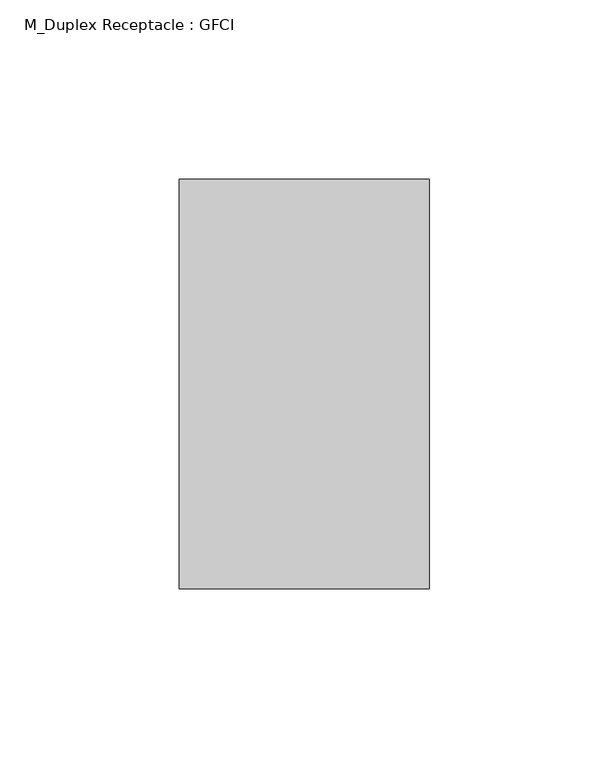
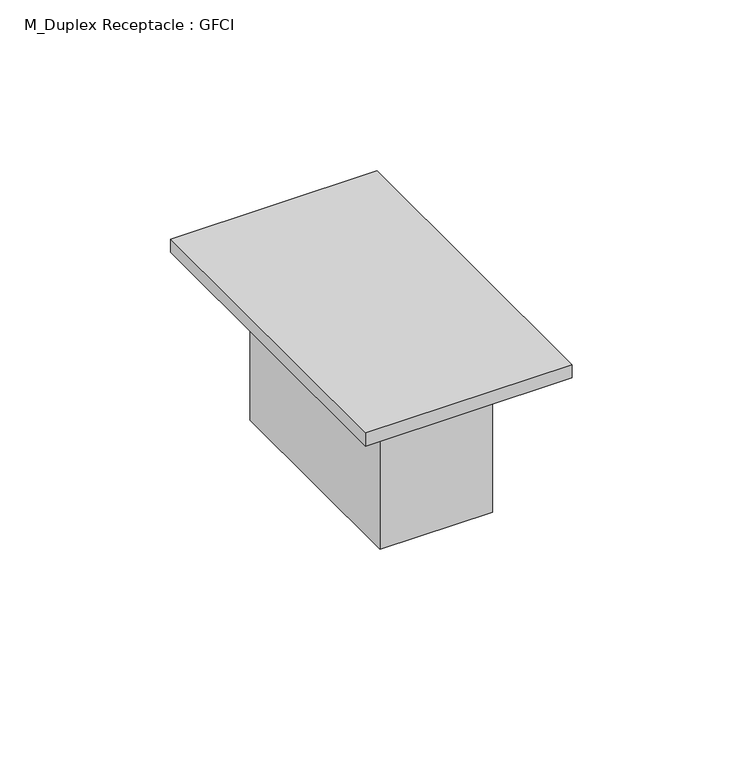
"""IFC4 building model written with IfcOpenShell, lengths in millimetres: proxy geometry, M_Duplex Receptacle : GFCI."""

from ifc_helpers import new_model, si_unit, frame, origin, origin_with_axes, place, context, project, spatial, polyline, outline, extrude, source, transform, mapped, element, save


def m_duplex_receptacle_gfci_367a9a66(model_context):
    return source(origin(), model_context, "Body", "SweptSolid", [
        extrude(outline(polyline([(34.925, 57.15), (34.925, -57.15), (-34.925, -57.15), (-34.925, 57.15), (34.925, 57.15)])), origin_with_axes(), (0.0, 0.0, 1.0), 4.7625),
        extrude(outline(polyline([(19.05, 38.1), (19.05, -38.1), (-19.05, -38.1), (-19.05, 38.1), (19.05, 38.1)])), frame((0.0, 0.0, -53.975), z_axis=(0.0, 0.0, 1.0), x_axis=(1.0, 0.0, 0.0)), (0.0, 0.0, 1.0), 53.975),
    ])


if __name__ == "__main__":
    model = new_model("IFC4")
    model_context = context("Model", 3, world=origin())
    ifc_project = project(units=[si_unit("LENGTHUNIT", "METRE", prefix="MILLI")], contexts=[model_context])
    site = spatial("IfcSite", under=ifc_project)
    building = spatial("IfcBuilding", under=site)
    placement = place(None, origin())
    m_duplex_receptacle_gfci_shape = m_duplex_receptacle_gfci_367a9a66(model_context)
    element("IfcBuildingElementProxy", 1, Name="M_Duplex Receptacle : GFCI", ObjectType="M_Duplex Receptacle : GFCI", at=placement, inside=building, context=model_context, shape_type="MappedRepresentation", body=[
        mapped(m_duplex_receptacle_gfci_shape, transform((0.0, 0.0, 0.0), x_axis=(1.0, 0.0, 0.0), y_axis=(0.0, 1.0, 0.0), z_axis=(0.0, 0.0, 1.0))),
    ])
    save(model, "model.ifc")

# Revit data of these elements
# Type "M_Duplex Receptacle : GFCI"
#   Label = "GFCI"
#   Switch Voltage = 120 V
#   Load = 180 VA
#   Default Elevation = 1.20 m
#   Load Classification = Receptacle
